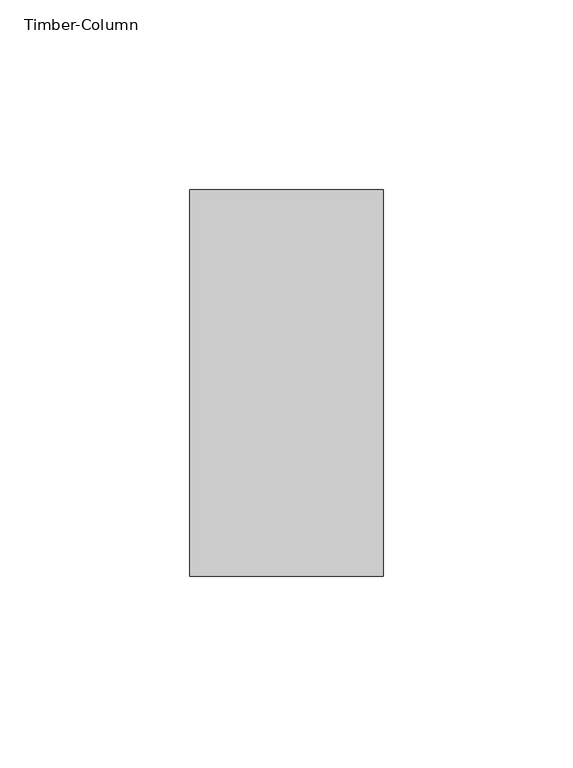
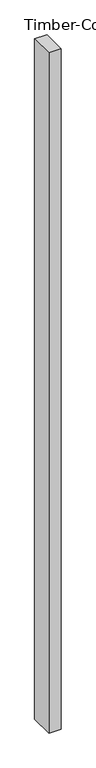
"""IFC4 building model written with IfcOpenShell, lengths in millimetres: column geometry, Timber-Column."""

from ifc_helpers import new_model, si_unit, frame, origin, place, context, project, spatial, polyline, outline, extrude, source, transform, mapped, element, save


def timber_column_4ee0a357(model_context):
    return source(origin(), model_context, "Body", "SweptSolid", [
        extrude(outline(polyline([(25.4, 50.8), (25.4, -50.8), (-25.4, -50.8), (-25.4, 50.8), (25.4, 50.8)])), frame((0.0, 0.0, -319.88125), z_axis=(0.0, 0.0, 1.0), x_axis=(1.0, 0.0, 0.0)), (0.0, 0.0, 1.0), 2986.88125),
    ])


if __name__ == "__main__":
    model = new_model("IFC4")
    model_context = context("Model", 3, world=origin())
    ifc_project = project(units=[si_unit("LENGTHUNIT", "METRE", prefix="MILLI")], contexts=[model_context])
    site = spatial("IfcSite", under=ifc_project)
    building = spatial("IfcBuilding", under=site)
    placement = place(None, origin())
    timber_column_shape = timber_column_4ee0a357(model_context)
    element("IfcColumn", 1, ObjectType="Timber-Column : BLDG 6241 Wall Struds 2\"x4\"", at=placement, inside=building, context=model_context, shape_type="MappedRepresentation", body=[
        mapped(timber_column_shape, transform((0.0, 0.0, 0.0), x_axis=(1.0, 0.0, 0.0), y_axis=(0.0, 1.0, 0.0), z_axis=(0.0, 0.0, 1.0))),
    ])
    save(model, "model.ifc")

# Revit data of these elements
# Type "Timber-Column : BLDG 6241 Wall Struds 2\"x4\""
#   Assembly Code = "B10"
#   A = 0.140625 SF
#   b = 0' - 2"
#   d = 0' - 4"
#   Structural Material [instance default] = Softwood, Lumber
# Element 1 (IfcColumn, "Timber-Column : BLDG 6241 Wall Struds 2\"x4\"")
#   Materials on its faces: "Softwood, Lumber"
# Materials
#   "Softwood, Lumber": class "Wood", colour RGB 223 192 134, transparency 0, Description = "Pinus Echinata", Cost = 0
